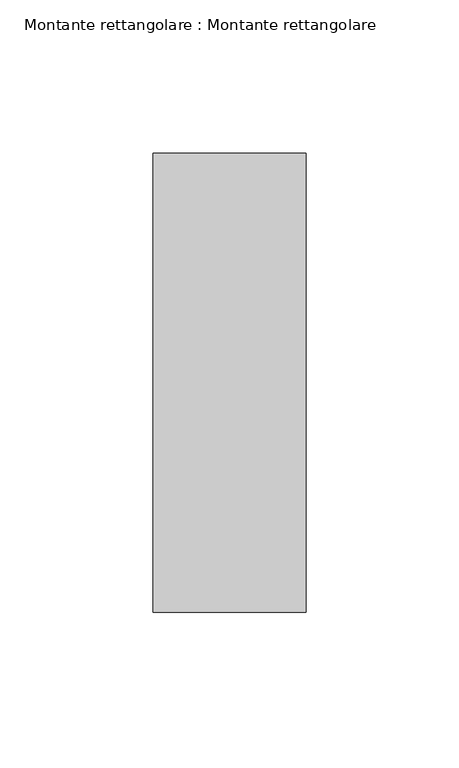
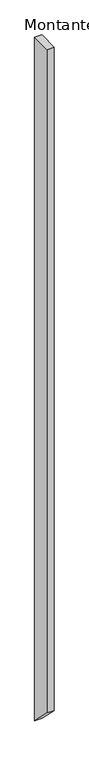
"""IFC4 building model written with IfcOpenShell, lengths in millimetres: member geometry, Montante rettangolare : Montante rettangolare."""

from ifc_helpers import new_model, si_unit, frame, origin, place, context, project, spatial, polyline, outline, extrude, source, transform, mapped, element, save


def montante_rettangolare_montante_rettangolare_ca0860d7(model_context):
    return source(origin(), model_context, "Body", "SweptSolid", [
        extrude(outline(polyline([(-75.0, 0.0), (75.0, 0.0), (75.0, -5080.0), (-75.0, -4930.0), (-75.0, 0.0)])), frame((-50.0, 0.0, 0.0), z_axis=(1.0, 0.0, 0.0), x_axis=(0.0, 1.0, 0.0)), (0.0, 0.0, 1.0), 50.0),
    ])


if __name__ == "__main__":
    model = new_model("IFC4")
    model_context = context("Model", 3, world=origin())
    ifc_project = project(units=[si_unit("LENGTHUNIT", "METRE", prefix="MILLI")], contexts=[model_context])
    site = spatial("IfcSite", under=ifc_project)
    building = spatial("IfcBuilding", under=site)
    placement = place(None, origin())
    montante_rettangolare_montante_rettangolare_shape = montante_rettangolare_montante_rettangolare_ca0860d7(model_context)
    element("IfcMember", 1, ObjectType="Montante rettangolare : Montante rettangolare", at=placement, inside=building, context=model_context, shape_type="MappedRepresentation", body=[
        mapped(montante_rettangolare_montante_rettangolare_shape, transform((0.0, 0.0, 0.0), x_axis=(1.0, 0.0, 0.0), y_axis=(0.0, 1.0, 0.0), z_axis=(0.0, 0.0, 1.0))),
    ])
    save(model, "model.ifc")

# Revit data of these elements
# Type "Montante rettangolare : Montante rettangolare"
#   built-in parameter 1007304 = 0.492126 (stored number, unit not read)
#   built-in parameter 1007301 = 0.082021 (stored number, unit not read)
#   built-in parameter 1007300 = 0.082021 (stored number, unit not read)
# Element 1 (IfcMember, "Montante rettangolare : Montante rettangolare")
#   Materials on its faces: "Acciaio"
# Materials
#   "Acciaio": class "Metallo", colour RGB 247 247 247, transparency 0, Description = "Acciaio, finitura zigrinata", Cost = 0
